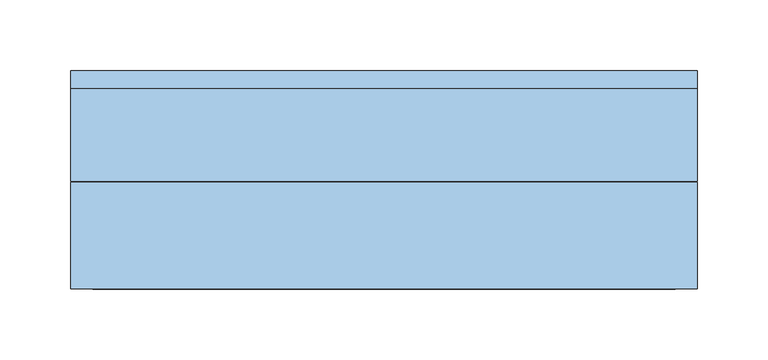
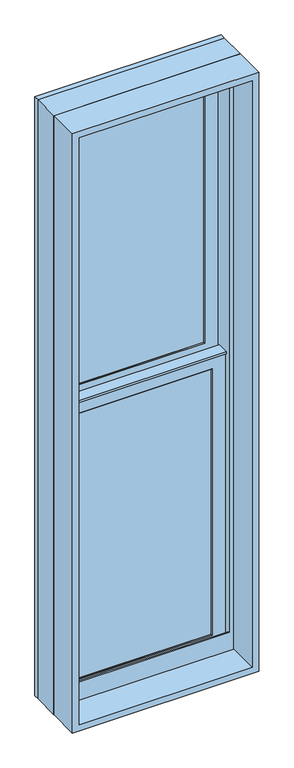
"""IFC4 building model written with IfcOpenShell, lengths in millimetres: window geometry, Window-Double_Hung-Marvin-Essential : ESDH1650."""

import ifcopenshell
import ifcopenshell.guid

model = None  # the IFC model being written
_history = None  # IfcOwnerHistory: only IFC2X3 demands one
_inside = {}  # id of a spatial element -> (the spatial element, [elements in it])
_under = {}  # id of a project, library or spatial element -> (it, [spatial elements below it])
_declared = {}  # id of a project -> (the project, [libraries it declares])
_typed = {}  # id of a type object -> (the type object, [elements of that type])
_made_of = {}  # id of a material, layer set ... -> (it, [elements and type objects made of it])


def new_model(schema):
    """Start an empty IFC model of exactly this schema.

    Asked for "IFC4X3", IfcOpenShell would pick the latest addendum, in which some entities
    have other attributes; the version numbers below select the first issue.
    IFC2X3 requires an IfcOwnerHistory on every rooted entity: one is made here for all.
    """
    global model, _history
    if schema == "IFC4X3":
        model = ifcopenshell.file(schema_version=(4, 3, 0, 0))
    else:
        model = ifcopenshell.file(schema=schema)
    _inside.clear()
    _under.clear()
    _declared.clear()
    _typed.clear()
    _made_of.clear()
    _history = None
    if model.schema == "IFC2X3":
        org = make("IfcOrganization", Name="unknown")
        user = make(
            "IfcPersonAndOrganization",
            ThePerson=make("IfcPerson", FamilyName="unknown"),
            TheOrganization=org,
        )
        app = make(
            "IfcApplication",
            ApplicationDeveloper=org,
            Version="unknown",
            ApplicationFullName="unknown",
            ApplicationIdentifier="unknown",
        )
        _history = make(
            "IfcOwnerHistory",
            OwningUser=user,
            OwningApplication=app,
            ChangeAction="ADDED",
            CreationDate=0,
        )
    return model


def make(cls, **values):
    """One entity of the class cls with the attributes given. An attribute that is None is left unset."""
    return model.create_entity(
        cls, **{name: value for name, value in values.items() if value is not None}
    )


def rooted(cls, **values):
    """An entity with a GlobalId (a new one), such as an element, a storey or a relation."""
    return make(cls, GlobalId=ifcopenshell.guid.new(), OwnerHistory=_history, **values)


def si_unit(unit_type, name, prefix=None):
    """IfcSIUnit, for example si_unit("LENGTHUNIT", "METRE", prefix="MILLI")."""
    return make("IfcSIUnit", UnitType=unit_type, Prefix=prefix, Name=name)


def assignment(units):
    """IfcUnitAssignment: the units of a project."""
    return None if units is None else make("IfcUnitAssignment", Units=units)


def point(xyz):
    """IfcCartesianPoint."""
    return None if xyz is None else make("IfcCartesianPoint", Coordinates=xyz)


def direction(xyz):
    """IfcDirection."""
    return None if xyz is None else make("IfcDirection", DirectionRatios=xyz)


def frame(location, z_axis=None, x_axis=None):
    """IfcAxis2Placement3D, a coordinate frame: its origin and axes. An axis left out is left unset."""
    return make(
        "IfcAxis2Placement3D",
        Location=point(location),
        Axis=direction(z_axis),
        RefDirection=direction(x_axis),
    )


def origin():
    """The frame at (0, 0, 0) with its axes left unset."""
    return frame((0.0, 0.0, 0.0))


def place(relative_to, where):
    """IfcLocalPlacement: puts the frame where relative to a parent placement (None: the world)."""
    return make(
        "IfcLocalPlacement", PlacementRelTo=relative_to, RelativePlacement=where
    )


def context(
    kind, dimensions, precision=None, world=None, true_north=None, identifier=None
):
    """IfcGeometricRepresentationContext, for example the 3D "Model" context."""
    return make(
        "IfcGeometricRepresentationContext",
        ContextIdentifier=identifier,
        ContextType=kind,
        CoordinateSpaceDimension=dimensions,
        Precision=precision,
        WorldCoordinateSystem=world,
        TrueNorth=true_north,
    )


def project(units=None, contexts=None):
    """IfcProject with its units and contexts."""
    return rooted(
        "IfcProject",
        Name="project",
        RepresentationContexts=contexts,
        UnitsInContext=assignment(units),
    )


def spatial(cls, under=None, at=None, **own):
    """A site, building, storey or space (cls), placed at a placement, below another one or the project."""
    s = rooted(cls, ObjectPlacement=at, **own)
    if under is not None:
        _under.setdefault(under.id(), (under, []))[1].append(s)
    return s


def polyline(points):
    """IfcPolyline through the points."""
    return make("IfcPolyline", Points=[point(p) for p in points])


def outline(outer, holes=None, kind="AREA"):
    """IfcArbitraryClosedProfileDef: a profile drawn as a closed curve; with holes, ...WithVoids."""
    if holes is None:
        return make("IfcArbitraryClosedProfileDef", ProfileType=kind, OuterCurve=outer)
    return make(
        "IfcArbitraryProfileDefWithVoids",
        ProfileType=kind,
        OuterCurve=outer,
        InnerCurves=holes,
    )


def extrude(swept, where, along, depth):
    """IfcExtrudedAreaSolid: the profile swept, set in the frame where, extruded along a direction by depth."""
    return make(
        "IfcExtrudedAreaSolid",
        SweptArea=swept,
        Position=where,
        ExtrudedDirection=direction(along),
        Depth=depth,
    )


def faces_of(points, faces, orient=None, outer=None):
    """IfcFace entities. A face is a list of loops; a loop is a list of indices into points, from 0.

    orient and outer hold one flag for each loop. By default every Orientation is true, the
    first loop of a face is its IfcFaceOuterBound and the others are IfcFaceBound.
    """
    made = []
    for i, loops in enumerate(faces):
        bounds = []
        for j, loop in enumerate(loops):
            is_outer = j == 0 if outer is None else outer[i][j]
            bounds.append(
                make(
                    "IfcFaceOuterBound" if is_outer else "IfcFaceBound",
                    Bound=make("IfcPolyLoop", Polygon=[points[k] for k in loop]),
                    Orientation=True if orient is None else orient[i][j],
                )
            )
        made.append(make("IfcFace", Bounds=bounds))
    return made


def faceted_brep(points, faces, orient=None, outer=None, voids=None):
    """IfcFacetedBrep: a solid bounded by flat faces; with voids (closed shells), ...WithVoids."""
    shared = [point(p) for p in points]
    hull = make("IfcClosedShell", CfsFaces=faces_of(shared, faces, orient, outer))
    if voids is None:
        return make("IfcFacetedBrep", Outer=hull)
    return make(
        "IfcFacetedBrepWithVoids",
        Outer=hull,
        Voids=[
            make(cls, CfsFaces=faces_of(shared, fs, o, b)) for cls, fs, o, b in voids
        ],
    )


def shape(context_of_items, identifier, shape_type, items):
    """IfcShapeRepresentation: the items that make up one representation, for example the "Body"."""
    return make(
        "IfcShapeRepresentation",
        ContextOfItems=context_of_items,
        RepresentationIdentifier=identifier,
        RepresentationType=shape_type,
        Items=items,
    )


def source(mapping_origin, context_of_items, identifier, shape_type, items):
    """IfcRepresentationMap: a shape defined once, which mapped items show again and again."""
    return make(
        "IfcRepresentationMap",
        MappingOrigin=mapping_origin,
        MappedRepresentation=shape(context_of_items, identifier, shape_type, items),
    )


def transform(
    local_origin,
    x_axis=None,
    y_axis=None,
    z_axis=None,
    scale=None,
    scale2=None,
    scale3=None,
    uniform=True,
):
    """IfcCartesianTransformationOperator3D, or its non-uniform kind. x_axis, y_axis, z_axis: its Axis1, 2, 3."""
    if uniform:
        return make(
            "IfcCartesianTransformationOperator3D",
            Axis1=direction(x_axis),
            Axis2=direction(y_axis),
            LocalOrigin=point(local_origin),
            Scale=scale,
            Axis3=direction(z_axis),
        )
    return make(
        "IfcCartesianTransformationOperator3DnonUniform",
        Axis1=direction(x_axis),
        Axis2=direction(y_axis),
        LocalOrigin=point(local_origin),
        Scale=scale,
        Axis3=direction(z_axis),
        Scale2=scale2,
        Scale3=scale3,
    )


def mapped(mapping_source, mapping_target):
    """IfcMappedItem: shows the shape of a source again, moved by a transform."""
    return make(
        "IfcMappedItem", MappingSource=mapping_source, MappingTarget=mapping_target
    )


def made_of(thing, what):
    """Note that an element or type object is made of a material, layer set ...; save() writes the relation."""
    if what is not None:
        _made_of.setdefault(what.id(), (what, []))[1].append(thing)
    return thing


def element(
    cls,
    number,
    at=None,
    inside=None,
    cuts=None,
    type_object=None,
    material=None,
    context=None,
    identifier="Body",
    shape_type=None,
    held_by="IfcProductDefinitionShape",
    body=None,
    shapes=None,
    **own,
):
    """One element of the class cls, such as IfcWall. Its Tag is "e" and its number.

    at: its placement. inside: the storey or other place that contains it. cuts: it is an
    opening in that element (IfcRelVoidsElement). A single representation is given by context,
    identifier, shape_type and body (its items); several are given by shapes. held_by: the class
    of the entity that holds the representations. save() writes the other relations.
    """
    e = rooted(cls, Tag="e%d" % number, ObjectPlacement=at, **own)
    if body is not None:
        shapes = [shape(context, identifier, shape_type, body)]
    if shapes is not None:
        e.Representation = make(held_by, Representations=shapes)
    if inside is not None:
        _inside.setdefault(inside.id(), (inside, []))[1].append(e)
    if cuts is not None:
        rooted(
            "IfcRelVoidsElement", RelatingBuildingElement=cuts, RelatedOpeningElement=e
        )
    if type_object is not None:
        _typed.setdefault(type_object.id(), (type_object, []))[1].append(e)
    return made_of(e, material)


def aggregate(whole, parts):
    """IfcRelAggregates: a whole, such as a stair, and the parts it consists of."""
    return rooted("IfcRelAggregates", RelatingObject=whole, RelatedObjects=parts)


def save(model, path):
    """Write the relations noted so far, then the file.

    IfcRelAggregates (storeys below a building ...), IfcRelContainedInSpatialStructure (elements
    in a storey), IfcRelDefinesByType, IfcRelAssociatesMaterial and IfcRelDeclares: one each for
    every whole, place, type object, material and project.
    """
    for whole, parts in _under.values():
        aggregate(whole, parts)
    for where, things in _inside.values():
        rooted(
            "IfcRelContainedInSpatialStructure",
            RelatedElements=things,
            RelatingStructure=where,
        )
    for kind, things in _typed.values():
        rooted("IfcRelDefinesByType", RelatedObjects=things, RelatingType=kind)
    for what, things in _made_of.values():
        rooted("IfcRelAssociatesMaterial", RelatedObjects=things, RelatingMaterial=what)
    for by, libraries in _declared.values():
        rooted("IfcRelDeclares", RelatingContext=by, RelatedDefinitions=libraries)
    model.write(path)


def window_373a512a(model_context):
    return source(origin(), model_context, "Body", "SolidModel", [
        extrude(outline(polyline([(64.5583333, 20.6375), (64.5583333, 15.875), (45.5083333, 15.875), (45.5083333, 20.6375), (64.5583333, 20.6375)])), frame((0.0, 0.0, 984.25), z_axis=(0.0, 0.0, 1.0), x_axis=(1.0, 0.0, 0.0)), (0.0, 0.0, 1.0), 679.45),
        extrude(outline(polyline([(-45.5083333, 20.6375), (-45.5083333, 15.875), (-64.5583333, 15.875), (-64.5583333, 20.6375), (-45.5083333, 20.6375)])), frame((0.0, 0.0, 984.25), z_axis=(0.0, 0.0, 1.0), x_axis=(1.0, 0.0, 0.0)), (0.0, 0.0, 1.0), 679.45),
        extrude(outline(polyline([(165.1, 20.6375), (165.1, 15.875), (-165.1, 15.875), (-165.1, 20.6375), (165.1, 20.6375)])), frame((0.0, 0.0, 1314.45), z_axis=(0.0, 0.0, 1.0), x_axis=(1.0, 0.0, 0.0)), (0.0, 0.0, 1.0), 19.05),
        extrude(outline(polyline([(-64.5583333, 46.83125), (-64.5583333, 51.59375), (-45.5083333, 51.59375), (-45.5083333, 46.83125), (-64.5583333, 46.83125)])), frame((0.0, 0.0, 1701.8), z_axis=(0.0, 0.0, 1.0), x_axis=(1.0, 0.0, 0.0)), (0.0, 0.0, 1.0), 679.45),
        extrude(outline(polyline([(45.5083333, 46.83125), (45.5083333, 51.59375), (64.5583333, 51.59375), (64.5583333, 46.83125), (45.5083333, 46.83125)])), frame((0.0, 0.0, 1701.8), z_axis=(0.0, 0.0, 1.0), x_axis=(1.0, 0.0, 0.0)), (0.0, 0.0, 1.0), 679.45),
        extrude(outline(polyline([(-165.1, 46.83125), (-165.1, 51.59375), (165.1, 51.59375), (165.1, 46.83125), (-165.1, 46.83125)])), frame((0.0, 0.0, 2032.0), z_axis=(0.0, 0.0, 1.0), x_axis=(1.0, 0.0, 0.0)), (0.0, 0.0, 1.0), 19.05),
        extrude(outline(polyline([(64.5583333, 20.6375), (45.5083333, 20.6375), (45.5083333, 25.4), (64.5583333, 25.4), (64.5583333, 20.6375)])), frame((0.0, 0.0, 984.25), z_axis=(0.0, 0.0, 1.0), x_axis=(1.0, 0.0, 0.0)), (0.0, 0.0, 1.0), 679.45),
        extrude(outline(polyline([(-45.5083333, 20.6375), (-64.5583333, 20.6375), (-64.5583333, 25.4), (-45.5083333, 25.4), (-45.5083333, 20.6375)])), frame((0.0, 0.0, 984.25), z_axis=(0.0, 0.0, 1.0), x_axis=(1.0, 0.0, 0.0)), (0.0, 0.0, 1.0), 679.45),
        extrude(outline(polyline([(165.1, 20.6375), (-165.1, 20.6375), (-165.1, 25.4), (165.1, 25.4), (165.1, 20.6375)])), frame((0.0, 0.0, 1314.45), z_axis=(0.0, 0.0, 1.0), x_axis=(1.0, 0.0, 0.0)), (0.0, 0.0, 1.0), 19.05),
        extrude(outline(polyline([(-64.5583333, 56.35625), (-45.5083333, 56.35625), (-45.5083333, 51.59375), (-64.5583333, 51.59375), (-64.5583333, 56.35625)])), frame((0.0, 0.0, 1701.8), z_axis=(0.0, 0.0, 1.0), x_axis=(1.0, 0.0, 0.0)), (0.0, 0.0, 1.0), 679.45),
        extrude(outline(polyline([(45.5083333, 56.35625), (64.5583333, 56.35625), (64.5583333, 51.59375), (45.5083333, 51.59375), (45.5083333, 56.35625)])), frame((0.0, 0.0, 1701.8), z_axis=(0.0, 0.0, 1.0), x_axis=(1.0, 0.0, 0.0)), (0.0, 0.0, 1.0), 679.45),
        extrude(outline(polyline([(-165.1, 56.35625), (165.1, 56.35625), (165.1, 51.59375), (-165.1, 51.59375), (-165.1, 56.35625)])), frame((0.0, 0.0, 2032.0), z_axis=(0.0, 0.0, 1.0), x_axis=(1.0, 0.0, 0.0)), (0.0, 0.0, 1.0), 19.05),
        faceted_brep([(-192.0875, 5.6780605, 1693.7351748), (-192.0875, 5.6780605, 1689.1), (192.0875, 5.6780605, 1689.1), (192.0875, 5.6780605, 1693.7351748), (-192.0875, 34.8118605, 1693.7351748), (192.0875, 34.8118605, 1693.7351748), (192.0875, 34.8118605, 1689.1), (-192.0875, 34.8118605, 1689.1), (-192.0875, 30.1625, 1689.1), (-192.0875, 30.1625, 957.2625), (-192.0875, 8.9241104, 957.2625), (-192.0875, 8.9241104, 1689.1), (192.0875, 8.9241104, 1689.1), (192.0875, 30.1625, 1689.1), (192.0875, 8.9241104, 957.2625), (192.0875, 30.1625, 957.2625), (-176.2034752, 11.90625, 1674.8034752), (-176.2034752, 30.1625, 1674.8034752), (176.2034752, 30.1625, 1674.8034752), (176.2034752, 11.90625, 1674.8034752), (-159.54375, 10.4662439, 1658.14375), (-159.54375, 11.90625, 1658.14375), (159.54375, 11.90625, 1658.14375), (159.54375, 10.4662439, 1658.14375), (161.0858834, 8.9241104, 1659.6858834), (-161.0858834, 8.9241104, 1659.6858834), (176.2034752, 30.1625, 973.1465248), (176.2034752, 11.90625, 973.1465248), (159.54375, 11.90625, 989.80625), (159.54375, 10.4662439, 989.80625), (161.0858834, 8.9241104, 988.2641166), (-176.2034752, 30.1625, 973.1465248), (-176.2034752, 11.90625, 973.1465248), (-159.54375, 11.90625, 989.80625), (-159.54375, 10.4662439, 989.80625), (-161.0858834, 8.9241104, 988.2641166)], [[[0, 1, 2, 3]], [[4, 5, 6, 7]], [[1, 0, 4, 7, 8, 9, 10, 11]], [[2, 1, 11, 12]], [[7, 6, 13, 8]], [[3, 2, 12, 14, 15, 13, 6, 5]], [[0, 3, 5, 4]], [[16, 17, 18, 19]], [[20, 21, 22, 23]], [[20, 23, 24, 25]], [[19, 18, 26, 27]], [[23, 22, 28, 29]], [[24, 23, 29, 30]], [[27, 26, 31, 32]], [[29, 28, 33, 34]], [[30, 29, 34, 35]], [[15, 14, 10, 9]], [[15, 9, 8, 13], [18, 17, 31, 26]], [[17, 16, 32, 31]], [[16, 19, 27, 32], [22, 21, 33, 28]], [[21, 20, 34, 33]], [[20, 25, 35, 34]], [[10, 14, 12, 11], [25, 24, 30, 35]]]),
        extrude(outline(polyline([(38.5955581, 1674.8125), (33.5778968, 1674.8125), (33.5778968, 1676.4), (39.9405976, 1676.4), (39.9405976, 1674.8125), (61.515625, 1674.8125), (47.6307501, 1671.4975159), (38.5955581, 1671.4975159), (38.5955581, 1674.8125)])), frame((-192.0875, 0.0, 0.0), z_axis=(1.0, 0.0, 0.0), x_axis=(0.0, 1.0, 0.0)), (0.0, 0.0, 1.0), 384.175),
        faceted_brep([(222.25, 0.0, 927.1), (222.25, 0.0, 2438.4), (-222.25, 0.0, 2438.4), (-222.25, 0.0, 927.1), (196.05625, 0.0, 988.21875), (-196.05625, 0.0, 988.21875), (-196.05625, 0.0, 2412.20625), (196.05625, 0.0, 2412.20625), (196.05625, 3.96875, 927.1), (-196.05625, 3.96875, 927.1), (-196.05625, 3.96875, 988.21875), (196.05625, 3.96875, 988.21875), (-222.25, 65.6828125, 927.1), (-196.05625, 65.6828125, 927.1), (196.05625, 65.6828125, 927.1), (222.25, 65.6828125, 927.1), (-222.25, 65.6828125, 2438.4), (222.25, 65.6828125, 2438.4), (196.05625, 65.6828125, 2412.20625), (-196.05625, 65.6828125, 2412.20625)], [[[0, 1, 2, 3], [4, 5, 6, 7]], [[8, 9, 10, 11]], [[5, 4, 11, 10]], [[0, 3, 12, 13, 9, 8, 14, 15]], [[13, 12, 16, 17, 15, 14, 18, 19]], [[13, 19, 6, 5, 10, 9]], [[7, 6, 19, 18]], [[18, 14, 8, 11, 4, 7]], [[1, 0, 15, 17]], [[2, 1, 17, 16]], [[3, 2, 16, 12]]]),
        faceted_brep([(196.05625, 30.1625, 1682.75), (194.46875, 30.1625, 1682.75), (194.46875, 30.1625, 951.4544613), (196.05625, 30.1625, 951.4544613), (-194.46875, 30.1625, 1682.75), (-196.05625, 30.1625, 1682.75), (-196.05625, 30.1625, 951.4544613), (-194.46875, 30.1625, 951.4544613), (194.46875, 63.5, 1682.75), (196.05625, 63.5, 1682.75), (196.05625, 63.5, 944.9743077), (194.46875, 63.5, 944.9743077), (-196.05625, 63.5, 1682.75), (-194.46875, 63.5, 1682.75), (-194.46875, 63.5, 944.9743077), (-196.05625, 63.5, 944.9743077), (207.3108932, 3.96875, 956.5460105), (207.3108932, 3.96875, 927.1), (207.3108932, 65.6828125, 927.1), (207.3108932, 65.6828125, 944.550012), (-207.3108932, 3.96875, 927.1), (-207.3108932, 3.96875, 956.5460105), (-207.3108932, 65.6828125, 944.550012), (-207.3108932, 65.6828125, 927.1), (207.3108932, 78.58125, 942.0428097), (-207.3108932, 78.58125, 942.0428097), (-205.2971252, 68.2348864, 944.0539391), (-187.33135, 68.2348864, 944.0539391), (-187.33135, 65.6828125, 944.550012), (187.33135, 65.6828125, 944.550012), (187.33135, 68.2348864, 944.0539391), (205.2971252, 68.2348864, 944.0539391), (-222.25, 65.6828125, 927.1), (-222.25, 78.5948249, 927.1), (222.25, 78.5948249, 927.1), (222.25, 65.6828125, 927.1), (-222.25, 78.58125, 2438.4), (222.25, 78.58125, 2438.4), (207.3108932, 78.58125, 2423.4608932), (-207.3108932, 78.58125, 2423.4608932), (-222.25, 65.6828125, 2438.4), (-205.2971252, 68.2348864, 2421.4471252), (205.2971252, 68.2348864, 2421.4471252), (187.33135, 68.2348864, 2403.48135), (-187.33135, 68.2348864, 2403.48135), (-187.33135, 65.6828125, 2403.48135), (187.33135, 65.6828125, 2403.48135), (222.25, 65.6828125, 2438.4)], [[[0, 1, 2, 3]], [[4, 5, 6, 7]], [[8, 9, 10, 11]], [[12, 13, 14, 15]], [[1, 8, 11, 2]], [[9, 0, 3, 10]], [[1, 0, 9, 8]], [[5, 4, 13, 12]], [[5, 12, 15, 6]], [[13, 4, 7, 14]], [[16, 17, 18, 19]], [[20, 21, 22, 23]], [[24, 25, 26, 27, 28, 22, 21, 16, 19, 29, 30, 31], [3, 2, 11, 10], [7, 6, 15, 14]], [[17, 16, 21, 20]], [[17, 20, 23, 32, 33, 34, 35, 18]], [[34, 33, 36, 37], [25, 24, 38, 39]], [[33, 32, 40, 36]], [[39, 41, 26, 25]], [[41, 42, 31, 30, 43, 44, 27, 26]], [[44, 45, 28, 27]], [[40, 32, 23, 22, 28, 45, 46, 29, 19, 18, 35, 47]], [[36, 40, 47, 37]], [[39, 38, 42, 41]], [[44, 43, 46, 45]], [[34, 37, 47, 35]], [[42, 38, 24, 31]], [[46, 43, 30, 29]]]),
        extrude(outline(polyline([(172.24375, 11.90625), (-172.24375, 11.90625), (-172.24375, 15.08125), (172.24375, 15.08125), (172.24375, 11.90625)])), frame((0.0, 0.0, 977.10625), z_axis=(0.0, 0.0, 1.0), x_axis=(1.0, 0.0, 0.0)), (0.0, 0.0, 1.0), 693.7375),
        extrude(outline(polyline([(172.24375, 42.8625), (-172.24375, 42.8625), (-172.24375, 46.0375), (172.24375, 46.0375), (172.24375, 42.8625)])), frame((0.0, 0.0, 1694.65625), z_axis=(0.0, 0.0, 1.0), x_axis=(1.0, 0.0, 0.0)), (0.0, 0.0, 1.0), 693.7375),
        faceted_brep([(-159.54375, 31.194477, 1658.14375), (-161.0858834, 32.7366104, 1659.6858834), (161.0858834, 32.7366104, 1659.6858834), (159.54375, 31.194477, 1658.14375), (-159.54375, 30.1625, 1658.14375), (159.54375, 30.1625, 1658.14375), (-192.0875, 32.7366104, 1690.6875), (-192.0875, 30.1625, 1690.6875), (192.0875, 30.1625, 1690.6875), (192.0875, 32.7366104, 1690.6875), (161.0858834, 32.7366104, 988.2641166), (159.54375, 31.194477, 989.80625), (159.54375, 30.1625, 989.80625), (192.0875, 30.1625, 957.2625), (192.0875, 32.7366104, 957.2625), (-161.0858834, 32.7366104, 988.2641166), (-159.54375, 31.194477, 989.80625), (-159.54375, 30.1625, 989.80625), (-192.0875, 30.1625, 957.2625), (-192.0875, 32.7366104, 957.2625)], [[[0, 1, 2, 3]], [[4, 0, 3, 5]], [[6, 7, 8, 9]], [[3, 2, 10, 11]], [[5, 3, 11, 12]], [[9, 8, 13, 14]], [[11, 10, 15, 16]], [[12, 11, 16, 17]], [[14, 13, 18, 19]], [[9, 14, 19, 6], [1, 15, 10, 2]], [[16, 15, 1, 0]], [[17, 16, 0, 4]], [[7, 18, 13, 8], [5, 12, 17, 4]], [[19, 18, 7, 6]]]),
        faceted_brep([(-176.2034752, 42.8625, 2392.3534752), (-176.2034752, 61.11875, 2392.3534752), (176.2034752, 61.11875, 2392.3534752), (176.2034752, 42.8625, 2392.3534752), (-159.54375, 41.4224939, 2375.69375), (-159.54375, 42.8625, 2375.69375), (159.54375, 42.8625, 2375.69375), (159.54375, 41.4224939, 2375.69375), (-161.0858834, 39.8803604, 2377.2358834), (161.0858834, 39.8803604, 2377.2358834), (-192.0875, 61.11875, 2408.2375), (-192.0875, 39.8803604, 2408.2375), (192.0875, 39.8803604, 2408.2375), (192.0875, 61.11875, 2408.2375), (176.2034752, 61.11875, 1690.6965248), (176.2034752, 42.8625, 1690.6965248), (159.54375, 42.8625, 1707.35625), (159.54375, 41.4224939, 1707.35625), (161.0858834, 39.8803604, 1705.8141166), (192.0875, 39.8803604, 1674.8125), (192.0875, 61.11875, 1674.8125), (-176.2034752, 61.11875, 1690.6965248), (-176.2034752, 42.8625, 1690.6965248), (-159.54375, 42.8625, 1707.35625), (-159.54375, 41.4224939, 1707.35625), (-161.0858834, 39.8803604, 1705.8141166), (-192.0875, 39.8803604, 1674.8125), (-192.0875, 61.11875, 1674.8125)], [[[0, 1, 2, 3]], [[4, 5, 6, 7]], [[8, 4, 7, 9]], [[10, 11, 12, 13]], [[3, 2, 14, 15]], [[7, 6, 16, 17]], [[9, 7, 17, 18]], [[13, 12, 19, 20]], [[15, 14, 21, 22]], [[17, 16, 23, 24]], [[18, 17, 24, 25]], [[20, 19, 26, 27]], [[13, 20, 27, 10], [1, 21, 14, 2]], [[22, 21, 1, 0]], [[3, 15, 22, 0], [5, 23, 16, 6]], [[24, 23, 5, 4]], [[25, 24, 4, 8]], [[11, 26, 19, 12], [9, 18, 25, 8]], [[27, 26, 11, 10]]]),
        faceted_brep([(-192.0875, 61.11875, 1674.8125), (-192.0875, 63.6928604, 1674.8125), (192.0875, 63.6928604, 1674.8125), (192.0875, 61.11875, 1674.8125), (-159.54375, 62.150727, 1707.35625), (-159.54375, 61.11875, 1707.35625), (159.54375, 61.11875, 1707.35625), (159.54375, 62.150727, 1707.35625), (-161.0858834, 63.6928604, 1705.8141166), (161.0858834, 63.6928604, 1705.8141166), (192.0875, 63.6928604, 2408.2375), (192.0875, 61.11875, 2408.2375), (159.54375, 61.11875, 2375.69375), (159.54375, 62.150727, 2375.69375), (161.0858834, 63.6928604, 2377.2358834), (-192.0875, 63.6928604, 2408.2375), (-192.0875, 61.11875, 2408.2375), (-159.54375, 61.11875, 2375.69375), (-159.54375, 62.150727, 2375.69375), (-161.0858834, 63.6928604, 2377.2358834)], [[[0, 1, 2, 3]], [[4, 5, 6, 7]], [[8, 4, 7, 9]], [[3, 2, 10, 11]], [[7, 6, 12, 13]], [[9, 7, 13, 14]], [[11, 10, 15, 16]], [[13, 12, 17, 18]], [[14, 13, 18, 19]], [[16, 15, 1, 0]], [[3, 11, 16, 0], [5, 17, 12, 6]], [[18, 17, 5, 4]], [[19, 18, 4, 8]], [[1, 15, 10, 2], [9, 14, 19, 8]]]),
        extrude(outline(polyline([(172.24375, 26.19375), (-172.24375, 26.19375), (-172.24375, 30.1625), (172.24375, 30.1625), (172.24375, 26.19375)])), frame((0.0, 0.0, 977.10625), z_axis=(0.0, 0.0, 1.0), x_axis=(1.0, 0.0, 0.0)), (0.0, 0.0, 1.0), 693.7375),
        extrude(outline(polyline([(172.24375, 57.15), (-172.24375, 57.15), (-172.24375, 61.11875), (172.24375, 61.11875), (172.24375, 57.15)])), frame((0.0, 0.0, 1694.65625), z_axis=(0.0, 0.0, 1.0), x_axis=(1.0, 0.0, 0.0)), (0.0, 0.0, 1.0), 693.7375),
        extrude(outline(polyline([(2438.4, 222.25), (2438.4, -222.25), (927.1, -222.25), (927.1, 222.25), (2438.4, 222.25)]), holes=[polyline([(2422.525, 206.375), (942.975, 206.375), (942.975, -206.375), (2422.525, -206.375), (2422.525, 206.375)])]), frame((0.0, -76.2, 0.0), z_axis=(0.0, 1.0, 0.0), x_axis=(0.0, 0.0, 1.0)), (0.0, 0.0, 1.0), 75.40625),
    ])


if __name__ == "__main__":
    model = new_model("IFC4")
    model_context = context("Model", 3, world=origin())
    ifc_project = project(units=[si_unit("LENGTHUNIT", "METRE", prefix="MILLI")], contexts=[model_context])
    site = spatial("IfcSite", under=ifc_project)
    building = spatial("IfcBuilding", under=site)
    placement = place(None, origin())
    window_shape = window_373a512a(model_context)
    element("IfcWindow", 1, ObjectType="Window-Double_Hung-Marvin-Essential : ESDH1650", at=placement, inside=building, context=model_context, shape_type="MappedRepresentation", body=[
        mapped(window_shape, transform((0.0, 0.0, 0.0), x_axis=(1.0, 0.0, 0.0), y_axis=(0.0, 1.0, 0.0), z_axis=(0.0, 0.0, 1.0))),
    ])
    save(model, "model.ifc")

# Revit data of these elements
# Type "Window-Double_Hung-Marvin-Essential : ESDH1650"
#   Type Mark = "61"
#   Window Type = "Essential Double Hung"
#   Product data url = "https://bimobject.com/marvin-windows-and-doors/product/marvin-dhwau"
#   Product Guid = "c4a96547-874c-4385-91dc-a058adc19d98"
#   Frame = "All Ultrex"
#   Egress Window = "No"
#   URL = "www.marvin.com"
#   Model = "ESDH1650"
#   Manufacturer = "Marvin Windows and Doors"
#   Label Egress = ""
#   Glass Type = "IG Low E II with Argon"
#   Design Pressure = "DP50"
#   Description = "1860 DBHG"
#   Analytic Construction = "<None>"
#   Prairie Corner Width = 0' - 4"
#   Prairie Corner Height = 0' - 4"
#   Egress Width = 1' - 2 9/16"
#   Egress Height = 2' - 1 27/128"
#   Rough Width = 1' - 6"
#   Rough Height = 5' - 0"
#   Nominal Width = 1' - 6"
#   Nominal Height = 5' - 0"
#   Inset to Installation Flange [instance default] = 0' - 1"
#   Height = 4' - 11 1/2"
#   Egress Area = 2.54954 SF
#   Default Head Height = 8' - 0"
#   Width = 1' - 5 1/2"
#   Daylight Area = 4.59098 SF
#   DLO Width = 1' - 0 9/16"
#   DLO Height = 2' - 2 5/16"
#   Muntins Top Sash = yes
#   Lites Wide Top Sash = 3
#   Lites Wide Bottom Sash = 3
#   Lites High Top Sash = 2
#   Lites High Bottom Sash = 2
#   Lite Cut Prairie 9 = no
#   Lite Cut HV Grid = yes
#   Muntins Bottom Sash = yes
#   Label Visibility = no
#   Jamb Extension Visibility = yes
#   Edition number = 1
#   Interior Material = Ultrex-Marvin-Stonewhite
#   Glazing Material = Glass-Marvin-IG Low E II with Argon
#   Cladding Material = Ultrex-Marvin-Pebblegray
#   Wall Closure = (empty or 0)
#   Assembly Code = ""
# Element 1 (IfcWindow, "Window-Double_Hung-Marvin-Essential : ESDH1650")
#   Materials on its faces: "Ultrex-Marvin-Pebblegray", "Ultrex-Marvin-Stonewhite", "Glass-Marvin-IG Low E II with Argon"
# Materials
#   "Ultrex-Marvin-Stonewhite": class "Paint", colour RGB 250 251 245, transparency 0
#   "Glass-Marvin-IG Low E II with Argon": class "Glass", colour RGB 0 128 192, transparency 0.85
#   "Ultrex-Marvin-Pebblegray": class "Paint", colour RGB 189 185 173, transparency 0
